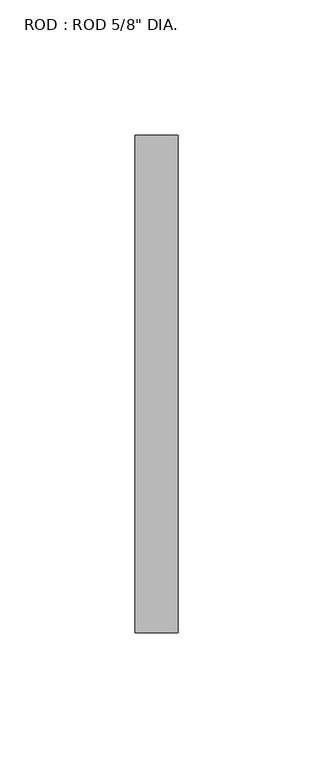
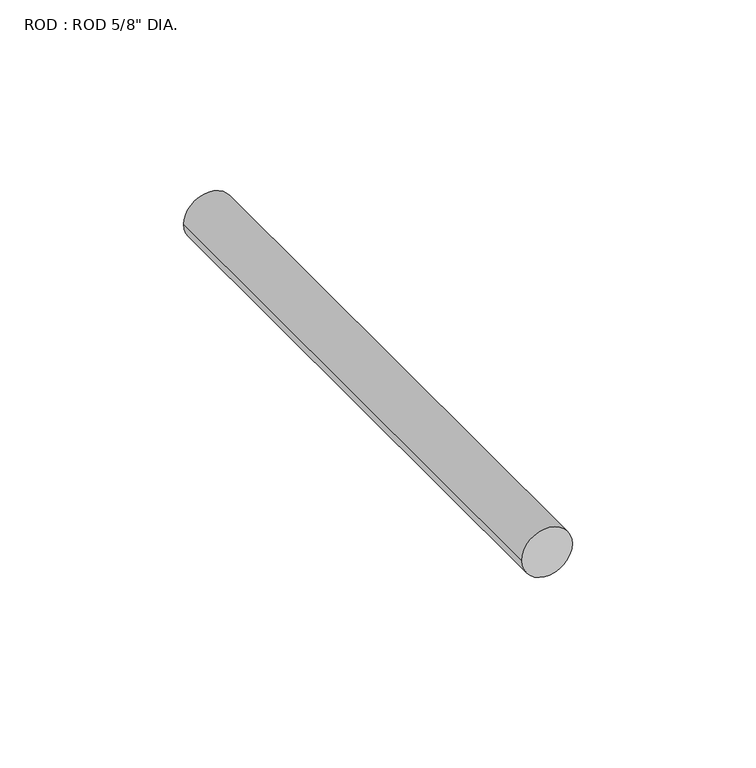
"""IFC4 building model written with IfcOpenShell, lengths in millimetres: proxy geometry."""

from ifc_helpers import new_model, si_unit, point, frame, origin, origin_2d, place, context, project, spatial, circle_curve, trimmed, segment, composite_curve, outline, extrude, source, transform, mapped, element, save


def proxy_760fde66(model_context):
    return source(origin(), model_context, "Body", "SweptSolid", [
        extrude(outline(composite_curve([segment(trimmed(circle_curve(origin_2d(), 7.9375), [point((0.0, 7.9375))], [point((0.0, -7.9375))], False, "CARTESIAN"), True, "CONTINUOUS"), segment(trimmed(circle_curve(origin_2d(), 7.9375), [point((0.0, -7.9375))], [point((0.0, 7.9375))], False, "CARTESIAN"), True, "CONTINUOUS")], self_intersect=False)), frame((0.0, -31.75, 0.0), z_axis=(0.0, 1.0, 0.0), x_axis=(0.0, 0.0, 1.0)), (0.0, 0.0, 1.0), 184.15),
    ])


if __name__ == "__main__":
    model = new_model("IFC4")
    model_context = context("Model", 3, world=origin())
    ifc_project = project(units=[si_unit("LENGTHUNIT", "METRE", prefix="MILLI")], contexts=[model_context])
    site = spatial("IfcSite", under=ifc_project)
    building = spatial("IfcBuilding", under=site)
    placement = place(None, origin())
    proxy_shape = proxy_760fde66(model_context)
    element("IfcBuildingElementProxy", 1, Name="ROD : ROD 5/8\" DIA.", ObjectType="ROD : ROD 5/8\" DIA.", at=placement, inside=building, context=model_context, shape_type="MappedRepresentation", body=[
        mapped(proxy_shape, transform((0.0, 0.0, 0.0), x_axis=(1.0, 0.0, 0.0), y_axis=(0.0, 1.0, 0.0), z_axis=(0.0, 0.0, 1.0))),
    ])
    save(model, "model.ifc")

# Revit data of these elements
# Type "ROD : ROD 5/8\" DIA."
#   lenght = 0' - 7 1/4"
#   Radius = 0' - 0 5/16"
#   material [instance default] = 3/4" GALV. THRU BOLTS
# Materials
#   "3/4\" GALV. THRU BOLTS": class "Generic", colour RGB 105 69 171, transparency 0, Cost = 0
